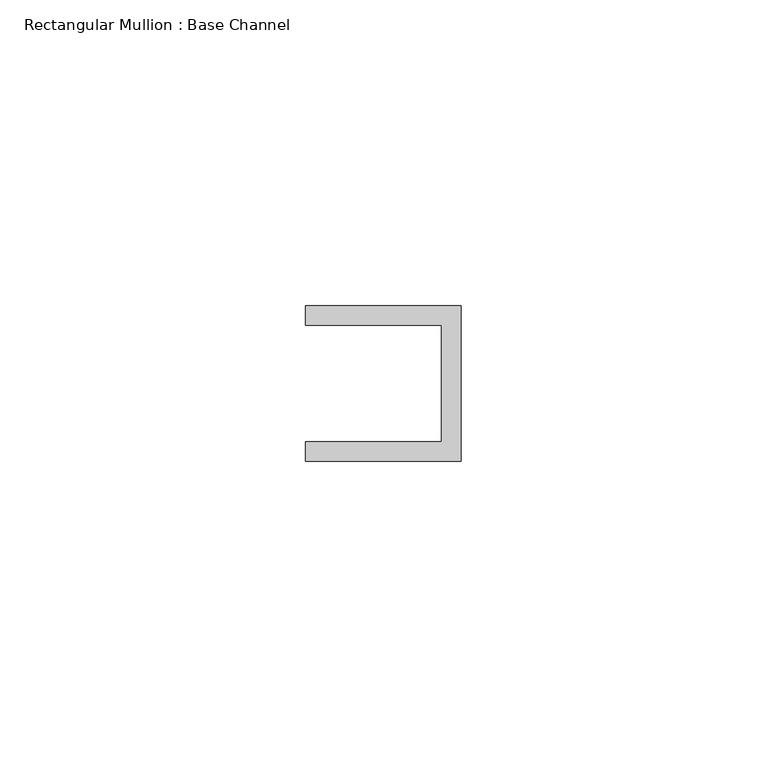
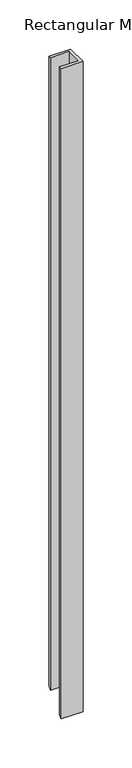
"""IFC4 building model written with IfcOpenShell, lengths in millimetres: member geometry, Rectangular Mullion : Base Channel."""

from ifc_helpers import new_model, si_unit, origin, place, context, project, spatial, faceted_brep, source, transform, mapped, element, save


def rectangular_mullion_base_channel_d69f46b3(model_context):
    return source(origin(), model_context, "Body", "Brep", [
        faceted_brep([(0.0, -12.7, 0.0), (0.0, 12.7, 0.0), (-25.4, 12.7, 0.0), (-25.4, 9.525, 0.0), (-3.175, 9.525, 0.0), (-3.175, -9.525, 0.0), (-25.4, -9.525, 0.0), (-25.4, -12.7, 0.0), (0.0, -12.7, -810.1591001), (0.0, 12.7, -784.7591001), (-25.4, 12.7, -784.7591001), (-25.4, 9.525, -787.9341001), (-3.175, 9.525, -787.9341001), (-3.175, -9.525, -806.9841001), (-25.4, -9.525, -806.9841001), (-25.4, -12.7, -810.1591001)], [[[0, 1, 2, 3, 4, 5, 6, 7]], [[1, 0, 8, 9]], [[2, 1, 9, 10]], [[3, 2, 10, 11]], [[4, 3, 11, 12]], [[5, 4, 12, 13]], [[6, 5, 13, 14]], [[7, 6, 14, 15]], [[0, 7, 15, 8]], [[8, 15, 14, 13, 12, 11, 10, 9]]]),
    ])


if __name__ == "__main__":
    model = new_model("IFC4")
    model_context = context("Model", 3, world=origin())
    ifc_project = project(units=[si_unit("LENGTHUNIT", "METRE", prefix="MILLI")], contexts=[model_context])
    site = spatial("IfcSite", under=ifc_project)
    building = spatial("IfcBuilding", under=site)
    placement = place(None, origin())
    rectangular_mullion_base_channel_shape = rectangular_mullion_base_channel_d69f46b3(model_context)
    element("IfcMember", 1, ObjectType="Rectangular Mullion : Base Channel", at=placement, inside=building, context=model_context, shape_type="MappedRepresentation", body=[
        mapped(rectangular_mullion_base_channel_shape, transform((0.0, 0.0, 0.0), x_axis=(1.0, 0.0, 0.0), y_axis=(0.0, 1.0, 0.0), z_axis=(0.0, 0.0, 1.0))),
    ])
    save(model, "model.ifc")

# Revit data of these elements
# Type "Rectangular Mullion : Base Channel"
#   built-in parameter 1007322 = 0.0833333 (stored number, unit not read)
#   built-in parameter 1007321 = 0.0416667 (stored number, unit not read)
#   built-in parameter 1007320 = -0.03125 (stored number, unit not read)
# Element 1 (IfcMember, "Rectangular Mullion : Base Channel")
#   Materials on its faces: "ALUM"
# Materials
#   "ALUM": class "Generic", colour RGB 157 157 157, transparency 0, Cost = 0
